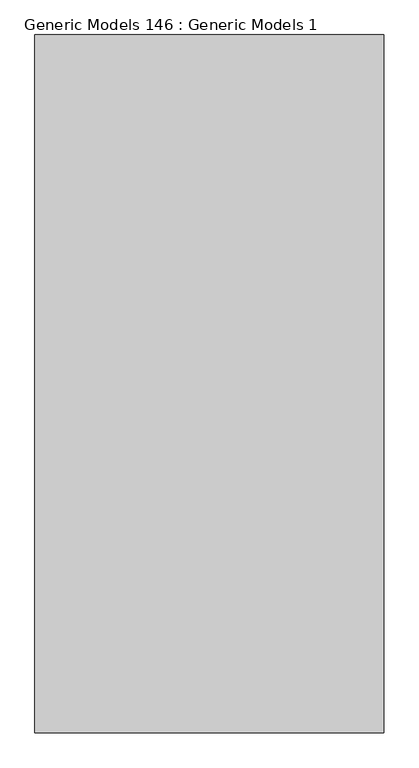
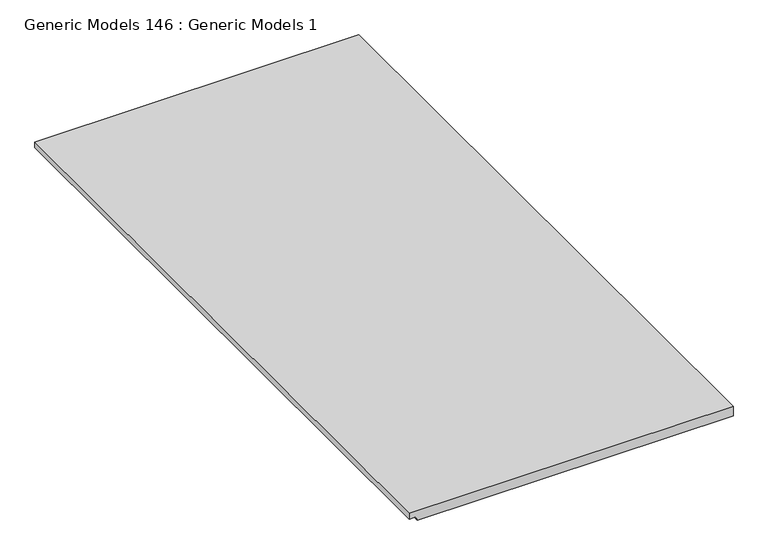
"""IFC4 building model written with IfcOpenShell, lengths in millimetres: proxy geometry, Generic Models 146 : Generic Models 1."""

import ifcopenshell
import ifcopenshell.guid

model = None  # the IFC model being written
_history = None  # IfcOwnerHistory: only IFC2X3 demands one
_inside = {}  # id of a spatial element -> (the spatial element, [elements in it])
_under = {}  # id of a project, library or spatial element -> (it, [spatial elements below it])
_declared = {}  # id of a project -> (the project, [libraries it declares])
_typed = {}  # id of a type object -> (the type object, [elements of that type])
_made_of = {}  # id of a material, layer set ... -> (it, [elements and type objects made of it])


def new_model(schema):
    """Start an empty IFC model of exactly this schema.

    Asked for "IFC4X3", IfcOpenShell would pick the latest addendum, in which some entities
    have other attributes; the version numbers below select the first issue.
    IFC2X3 requires an IfcOwnerHistory on every rooted entity: one is made here for all.
    """
    global model, _history
    if schema == "IFC4X3":
        model = ifcopenshell.file(schema_version=(4, 3, 0, 0))
    else:
        model = ifcopenshell.file(schema=schema)
    _inside.clear()
    _under.clear()
    _declared.clear()
    _typed.clear()
    _made_of.clear()
    _history = None
    if model.schema == "IFC2X3":
        org = make("IfcOrganization", Name="unknown")
        user = make(
            "IfcPersonAndOrganization",
            ThePerson=make("IfcPerson", FamilyName="unknown"),
            TheOrganization=org,
        )
        app = make(
            "IfcApplication",
            ApplicationDeveloper=org,
            Version="unknown",
            ApplicationFullName="unknown",
            ApplicationIdentifier="unknown",
        )
        _history = make(
            "IfcOwnerHistory",
            OwningUser=user,
            OwningApplication=app,
            ChangeAction="ADDED",
            CreationDate=0,
        )
    return model


def make(cls, **values):
    """One entity of the class cls with the attributes given. An attribute that is None is left unset."""
    return model.create_entity(
        cls, **{name: value for name, value in values.items() if value is not None}
    )


def rooted(cls, **values):
    """An entity with a GlobalId (a new one), such as an element, a storey or a relation."""
    return make(cls, GlobalId=ifcopenshell.guid.new(), OwnerHistory=_history, **values)


def si_unit(unit_type, name, prefix=None):
    """IfcSIUnit, for example si_unit("LENGTHUNIT", "METRE", prefix="MILLI")."""
    return make("IfcSIUnit", UnitType=unit_type, Prefix=prefix, Name=name)


def assignment(units):
    """IfcUnitAssignment: the units of a project."""
    return None if units is None else make("IfcUnitAssignment", Units=units)


def point(xyz):
    """IfcCartesianPoint."""
    return None if xyz is None else make("IfcCartesianPoint", Coordinates=xyz)


def direction(xyz):
    """IfcDirection."""
    return None if xyz is None else make("IfcDirection", DirectionRatios=xyz)


def frame(location, z_axis=None, x_axis=None):
    """IfcAxis2Placement3D, a coordinate frame: its origin and axes. An axis left out is left unset."""
    return make(
        "IfcAxis2Placement3D",
        Location=point(location),
        Axis=direction(z_axis),
        RefDirection=direction(x_axis),
    )


def origin():
    """The frame at (0, 0, 0) with its axes left unset."""
    return frame((0.0, 0.0, 0.0))


def place(relative_to, where):
    """IfcLocalPlacement: puts the frame where relative to a parent placement (None: the world)."""
    return make(
        "IfcLocalPlacement", PlacementRelTo=relative_to, RelativePlacement=where
    )


def context(
    kind, dimensions, precision=None, world=None, true_north=None, identifier=None
):
    """IfcGeometricRepresentationContext, for example the 3D "Model" context."""
    return make(
        "IfcGeometricRepresentationContext",
        ContextIdentifier=identifier,
        ContextType=kind,
        CoordinateSpaceDimension=dimensions,
        Precision=precision,
        WorldCoordinateSystem=world,
        TrueNorth=true_north,
    )


def project(units=None, contexts=None):
    """IfcProject with its units and contexts."""
    return rooted(
        "IfcProject",
        Name="project",
        RepresentationContexts=contexts,
        UnitsInContext=assignment(units),
    )


def spatial(cls, under=None, at=None, **own):
    """A site, building, storey or space (cls), placed at a placement, below another one or the project."""
    s = rooted(cls, ObjectPlacement=at, **own)
    if under is not None:
        _under.setdefault(under.id(), (under, []))[1].append(s)
    return s


def polyline(points):
    """IfcPolyline through the points."""
    return make("IfcPolyline", Points=[point(p) for p in points])


def outline(outer, holes=None, kind="AREA"):
    """IfcArbitraryClosedProfileDef: a profile drawn as a closed curve; with holes, ...WithVoids."""
    if holes is None:
        return make("IfcArbitraryClosedProfileDef", ProfileType=kind, OuterCurve=outer)
    return make(
        "IfcArbitraryProfileDefWithVoids",
        ProfileType=kind,
        OuterCurve=outer,
        InnerCurves=holes,
    )


def extrude(swept, where, along, depth):
    """IfcExtrudedAreaSolid: the profile swept, set in the frame where, extruded along a direction by depth."""
    return make(
        "IfcExtrudedAreaSolid",
        SweptArea=swept,
        Position=where,
        ExtrudedDirection=direction(along),
        Depth=depth,
    )


def shape(context_of_items, identifier, shape_type, items):
    """IfcShapeRepresentation: the items that make up one representation, for example the "Body"."""
    return make(
        "IfcShapeRepresentation",
        ContextOfItems=context_of_items,
        RepresentationIdentifier=identifier,
        RepresentationType=shape_type,
        Items=items,
    )


def source(mapping_origin, context_of_items, identifier, shape_type, items):
    """IfcRepresentationMap: a shape defined once, which mapped items show again and again."""
    return make(
        "IfcRepresentationMap",
        MappingOrigin=mapping_origin,
        MappedRepresentation=shape(context_of_items, identifier, shape_type, items),
    )


def transform(
    local_origin,
    x_axis=None,
    y_axis=None,
    z_axis=None,
    scale=None,
    scale2=None,
    scale3=None,
    uniform=True,
):
    """IfcCartesianTransformationOperator3D, or its non-uniform kind. x_axis, y_axis, z_axis: its Axis1, 2, 3."""
    if uniform:
        return make(
            "IfcCartesianTransformationOperator3D",
            Axis1=direction(x_axis),
            Axis2=direction(y_axis),
            LocalOrigin=point(local_origin),
            Scale=scale,
            Axis3=direction(z_axis),
        )
    return make(
        "IfcCartesianTransformationOperator3DnonUniform",
        Axis1=direction(x_axis),
        Axis2=direction(y_axis),
        LocalOrigin=point(local_origin),
        Scale=scale,
        Axis3=direction(z_axis),
        Scale2=scale2,
        Scale3=scale3,
    )


def mapped(mapping_source, mapping_target):
    """IfcMappedItem: shows the shape of a source again, moved by a transform."""
    return make(
        "IfcMappedItem", MappingSource=mapping_source, MappingTarget=mapping_target
    )


def made_of(thing, what):
    """Note that an element or type object is made of a material, layer set ...; save() writes the relation."""
    if what is not None:
        _made_of.setdefault(what.id(), (what, []))[1].append(thing)
    return thing


def element(
    cls,
    number,
    at=None,
    inside=None,
    cuts=None,
    type_object=None,
    material=None,
    context=None,
    identifier="Body",
    shape_type=None,
    held_by="IfcProductDefinitionShape",
    body=None,
    shapes=None,
    **own,
):
    """One element of the class cls, such as IfcWall. Its Tag is "e" and its number.

    at: its placement. inside: the storey or other place that contains it. cuts: it is an
    opening in that element (IfcRelVoidsElement). A single representation is given by context,
    identifier, shape_type and body (its items); several are given by shapes. held_by: the class
    of the entity that holds the representations. save() writes the other relations.
    """
    e = rooted(cls, Tag="e%d" % number, ObjectPlacement=at, **own)
    if body is not None:
        shapes = [shape(context, identifier, shape_type, body)]
    if shapes is not None:
        e.Representation = make(held_by, Representations=shapes)
    if inside is not None:
        _inside.setdefault(inside.id(), (inside, []))[1].append(e)
    if cuts is not None:
        rooted(
            "IfcRelVoidsElement", RelatingBuildingElement=cuts, RelatedOpeningElement=e
        )
    if type_object is not None:
        _typed.setdefault(type_object.id(), (type_object, []))[1].append(e)
    return made_of(e, material)


def aggregate(whole, parts):
    """IfcRelAggregates: a whole, such as a stair, and the parts it consists of."""
    return rooted("IfcRelAggregates", RelatingObject=whole, RelatedObjects=parts)


def save(model, path):
    """Write the relations noted so far, then the file.

    IfcRelAggregates (storeys below a building ...), IfcRelContainedInSpatialStructure (elements
    in a storey), IfcRelDefinesByType, IfcRelAssociatesMaterial and IfcRelDeclares: one each for
    every whole, place, type object, material and project.
    """
    for whole, parts in _under.values():
        aggregate(whole, parts)
    for where, things in _inside.values():
        rooted(
            "IfcRelContainedInSpatialStructure",
            RelatedElements=things,
            RelatingStructure=where,
        )
    for kind, things in _typed.values():
        rooted("IfcRelDefinesByType", RelatedObjects=things, RelatingType=kind)
    for what, things in _made_of.values():
        rooted("IfcRelAssociatesMaterial", RelatedObjects=things, RelatingMaterial=what)
    for by, libraries in _declared.values():
        rooted("IfcRelDeclares", RelatingContext=by, RelatedDefinitions=libraries)
    model.write(path)


def generic_models_146_generic_models_1_64768bb5(model_context):
    return source(origin(), model_context, "Body", "SweptSolid", [
        extrude(outline(polyline([(2027.354361, 46965.2186938), (2016.241861, 46965.2186938), (2016.241861, 46977.9186938), (2008.304361, 46980.8077075), (2008.304361, 47574.8186938), (2027.354361, 47574.8186938), (2027.354361, 46965.2186938)])), frame((0.0, 0.0, 0.0), z_axis=(0.0, 1.0, 0.0), x_axis=(0.0, 0.0, 1.0)), (0.0, 0.0, 1.0), 1219.2),
    ])


if __name__ == "__main__":
    model = new_model("IFC4")
    model_context = context("Model", 3, world=origin())
    ifc_project = project(units=[si_unit("LENGTHUNIT", "METRE", prefix="MILLI")], contexts=[model_context])
    site = spatial("IfcSite", under=ifc_project)
    building = spatial("IfcBuilding", under=site)
    placement = place(None, origin())
    generic_models_146_generic_models_1_shape = generic_models_146_generic_models_1_64768bb5(model_context)
    element("IfcBuildingElementProxy", 1, Name="Generic Models 146 : Generic Models 1", ObjectType="Generic Models 146 : Generic Models 1", at=placement, inside=building, context=model_context, shape_type="MappedRepresentation", body=[
        mapped(generic_models_146_generic_models_1_shape, transform((0.0, 0.0, 0.0), x_axis=(1.0, 0.0, 0.0), y_axis=(0.0, 1.0, 0.0), z_axis=(0.0, 0.0, 1.0))),
    ])
    save(model, "model.ifc")

# Revit data of these elements
# Element 1 (IfcBuildingElementProxy, "Generic Models 146 : Generic Models 1")
#   Materials on its faces: "CEILING AS SCHEDULED"
# Materials
#   "CEILING AS SCHEDULED": class "Generic", colour RGB 255 255 255, transparency 0, Cost = 0
